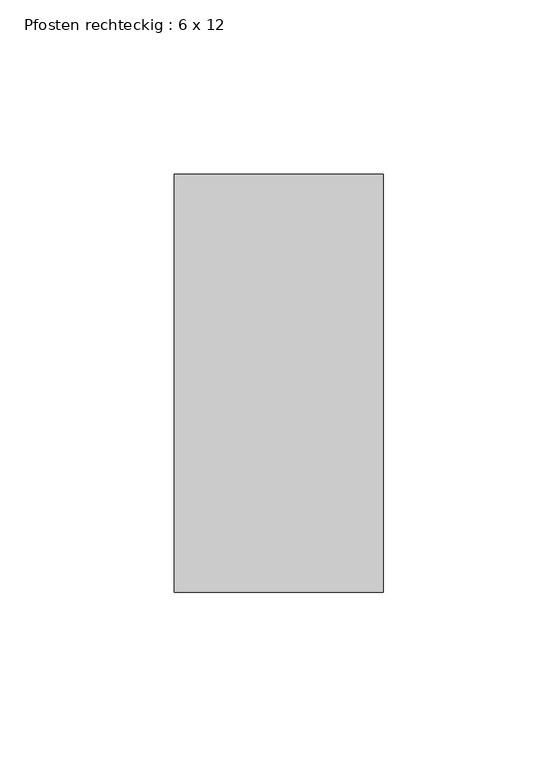
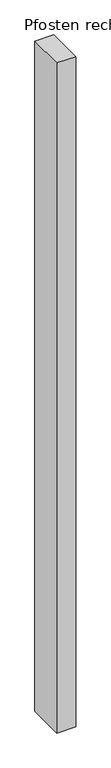
"""IFC4 building model written with IfcOpenShell, lengths in millimetres: member geometry, Pfosten rechteckig : 6 x 12."""

import ifcopenshell
import ifcopenshell.guid

model = None  # the IFC model being written
_history = None  # IfcOwnerHistory: only IFC2X3 demands one
_inside = {}  # id of a spatial element -> (the spatial element, [elements in it])
_under = {}  # id of a project, library or spatial element -> (it, [spatial elements below it])
_declared = {}  # id of a project -> (the project, [libraries it declares])
_typed = {}  # id of a type object -> (the type object, [elements of that type])
_made_of = {}  # id of a material, layer set ... -> (it, [elements and type objects made of it])


def new_model(schema):
    """Start an empty IFC model of exactly this schema.

    Asked for "IFC4X3", IfcOpenShell would pick the latest addendum, in which some entities
    have other attributes; the version numbers below select the first issue.
    IFC2X3 requires an IfcOwnerHistory on every rooted entity: one is made here for all.
    """
    global model, _history
    if schema == "IFC4X3":
        model = ifcopenshell.file(schema_version=(4, 3, 0, 0))
    else:
        model = ifcopenshell.file(schema=schema)
    _inside.clear()
    _under.clear()
    _declared.clear()
    _typed.clear()
    _made_of.clear()
    _history = None
    if model.schema == "IFC2X3":
        org = make("IfcOrganization", Name="unknown")
        user = make(
            "IfcPersonAndOrganization",
            ThePerson=make("IfcPerson", FamilyName="unknown"),
            TheOrganization=org,
        )
        app = make(
            "IfcApplication",
            ApplicationDeveloper=org,
            Version="unknown",
            ApplicationFullName="unknown",
            ApplicationIdentifier="unknown",
        )
        _history = make(
            "IfcOwnerHistory",
            OwningUser=user,
            OwningApplication=app,
            ChangeAction="ADDED",
            CreationDate=0,
        )
    return model


def make(cls, **values):
    """One entity of the class cls with the attributes given. An attribute that is None is left unset."""
    return model.create_entity(
        cls, **{name: value for name, value in values.items() if value is not None}
    )


def rooted(cls, **values):
    """An entity with a GlobalId (a new one), such as an element, a storey or a relation."""
    return make(cls, GlobalId=ifcopenshell.guid.new(), OwnerHistory=_history, **values)


def si_unit(unit_type, name, prefix=None):
    """IfcSIUnit, for example si_unit("LENGTHUNIT", "METRE", prefix="MILLI")."""
    return make("IfcSIUnit", UnitType=unit_type, Prefix=prefix, Name=name)


def assignment(units):
    """IfcUnitAssignment: the units of a project."""
    return None if units is None else make("IfcUnitAssignment", Units=units)


def point(xyz):
    """IfcCartesianPoint."""
    return None if xyz is None else make("IfcCartesianPoint", Coordinates=xyz)


def direction(xyz):
    """IfcDirection."""
    return None if xyz is None else make("IfcDirection", DirectionRatios=xyz)


def frame(location, z_axis=None, x_axis=None):
    """IfcAxis2Placement3D, a coordinate frame: its origin and axes. An axis left out is left unset."""
    return make(
        "IfcAxis2Placement3D",
        Location=point(location),
        Axis=direction(z_axis),
        RefDirection=direction(x_axis),
    )


def origin():
    """The frame at (0, 0, 0) with its axes left unset."""
    return frame((0.0, 0.0, 0.0))


def place(relative_to, where):
    """IfcLocalPlacement: puts the frame where relative to a parent placement (None: the world)."""
    return make(
        "IfcLocalPlacement", PlacementRelTo=relative_to, RelativePlacement=where
    )


def context(
    kind, dimensions, precision=None, world=None, true_north=None, identifier=None
):
    """IfcGeometricRepresentationContext, for example the 3D "Model" context."""
    return make(
        "IfcGeometricRepresentationContext",
        ContextIdentifier=identifier,
        ContextType=kind,
        CoordinateSpaceDimension=dimensions,
        Precision=precision,
        WorldCoordinateSystem=world,
        TrueNorth=true_north,
    )


def project(units=None, contexts=None):
    """IfcProject with its units and contexts."""
    return rooted(
        "IfcProject",
        Name="project",
        RepresentationContexts=contexts,
        UnitsInContext=assignment(units),
    )


def spatial(cls, under=None, at=None, **own):
    """A site, building, storey or space (cls), placed at a placement, below another one or the project."""
    s = rooted(cls, ObjectPlacement=at, **own)
    if under is not None:
        _under.setdefault(under.id(), (under, []))[1].append(s)
    return s


def polyline(points):
    """IfcPolyline through the points."""
    return make("IfcPolyline", Points=[point(p) for p in points])


def outline(outer, holes=None, kind="AREA"):
    """IfcArbitraryClosedProfileDef: a profile drawn as a closed curve; with holes, ...WithVoids."""
    if holes is None:
        return make("IfcArbitraryClosedProfileDef", ProfileType=kind, OuterCurve=outer)
    return make(
        "IfcArbitraryProfileDefWithVoids",
        ProfileType=kind,
        OuterCurve=outer,
        InnerCurves=holes,
    )


def extrude(swept, where, along, depth):
    """IfcExtrudedAreaSolid: the profile swept, set in the frame where, extruded along a direction by depth."""
    return make(
        "IfcExtrudedAreaSolid",
        SweptArea=swept,
        Position=where,
        ExtrudedDirection=direction(along),
        Depth=depth,
    )


def shape(context_of_items, identifier, shape_type, items):
    """IfcShapeRepresentation: the items that make up one representation, for example the "Body"."""
    return make(
        "IfcShapeRepresentation",
        ContextOfItems=context_of_items,
        RepresentationIdentifier=identifier,
        RepresentationType=shape_type,
        Items=items,
    )


def source(mapping_origin, context_of_items, identifier, shape_type, items):
    """IfcRepresentationMap: a shape defined once, which mapped items show again and again."""
    return make(
        "IfcRepresentationMap",
        MappingOrigin=mapping_origin,
        MappedRepresentation=shape(context_of_items, identifier, shape_type, items),
    )


def transform(
    local_origin,
    x_axis=None,
    y_axis=None,
    z_axis=None,
    scale=None,
    scale2=None,
    scale3=None,
    uniform=True,
):
    """IfcCartesianTransformationOperator3D, or its non-uniform kind. x_axis, y_axis, z_axis: its Axis1, 2, 3."""
    if uniform:
        return make(
            "IfcCartesianTransformationOperator3D",
            Axis1=direction(x_axis),
            Axis2=direction(y_axis),
            LocalOrigin=point(local_origin),
            Scale=scale,
            Axis3=direction(z_axis),
        )
    return make(
        "IfcCartesianTransformationOperator3DnonUniform",
        Axis1=direction(x_axis),
        Axis2=direction(y_axis),
        LocalOrigin=point(local_origin),
        Scale=scale,
        Axis3=direction(z_axis),
        Scale2=scale2,
        Scale3=scale3,
    )


def mapped(mapping_source, mapping_target):
    """IfcMappedItem: shows the shape of a source again, moved by a transform."""
    return make(
        "IfcMappedItem", MappingSource=mapping_source, MappingTarget=mapping_target
    )


def made_of(thing, what):
    """Note that an element or type object is made of a material, layer set ...; save() writes the relation."""
    if what is not None:
        _made_of.setdefault(what.id(), (what, []))[1].append(thing)
    return thing


def element(
    cls,
    number,
    at=None,
    inside=None,
    cuts=None,
    type_object=None,
    material=None,
    context=None,
    identifier="Body",
    shape_type=None,
    held_by="IfcProductDefinitionShape",
    body=None,
    shapes=None,
    **own,
):
    """One element of the class cls, such as IfcWall. Its Tag is "e" and its number.

    at: its placement. inside: the storey or other place that contains it. cuts: it is an
    opening in that element (IfcRelVoidsElement). A single representation is given by context,
    identifier, shape_type and body (its items); several are given by shapes. held_by: the class
    of the entity that holds the representations. save() writes the other relations.
    """
    e = rooted(cls, Tag="e%d" % number, ObjectPlacement=at, **own)
    if body is not None:
        shapes = [shape(context, identifier, shape_type, body)]
    if shapes is not None:
        e.Representation = make(held_by, Representations=shapes)
    if inside is not None:
        _inside.setdefault(inside.id(), (inside, []))[1].append(e)
    if cuts is not None:
        rooted(
            "IfcRelVoidsElement", RelatingBuildingElement=cuts, RelatedOpeningElement=e
        )
    if type_object is not None:
        _typed.setdefault(type_object.id(), (type_object, []))[1].append(e)
    return made_of(e, material)


def aggregate(whole, parts):
    """IfcRelAggregates: a whole, such as a stair, and the parts it consists of."""
    return rooted("IfcRelAggregates", RelatingObject=whole, RelatedObjects=parts)


def save(model, path):
    """Write the relations noted so far, then the file.

    IfcRelAggregates (storeys below a building ...), IfcRelContainedInSpatialStructure (elements
    in a storey), IfcRelDefinesByType, IfcRelAssociatesMaterial and IfcRelDeclares: one each for
    every whole, place, type object, material and project.
    """
    for whole, parts in _under.values():
        aggregate(whole, parts)
    for where, things in _inside.values():
        rooted(
            "IfcRelContainedInSpatialStructure",
            RelatedElements=things,
            RelatingStructure=where,
        )
    for kind, things in _typed.values():
        rooted("IfcRelDefinesByType", RelatedObjects=things, RelatingType=kind)
    for what, things in _made_of.values():
        rooted("IfcRelAssociatesMaterial", RelatedObjects=things, RelatingMaterial=what)
    for by, libraries in _declared.values():
        rooted("IfcRelDeclares", RelatingContext=by, RelatedDefinitions=libraries)
    model.write(path)


def pfosten_rechteckig_6_x_12_8f909f43(model_context):
    return source(origin(), model_context, "Body", "SweptSolid", [
        extrude(outline(polyline([(30.0, 60.0), (30.0, -60.0), (-30.0, -60.0), (-30.0, 60.0), (30.0, 60.0)])), frame((0.0, 0.0, -2250.0), z_axis=(0.0, 0.0, 1.0), x_axis=(1.0, 0.0, 0.0)), (0.0, 0.0, 1.0), 2250.0),
    ])


if __name__ == "__main__":
    model = new_model("IFC4")
    model_context = context("Model", 3, world=origin())
    ifc_project = project(units=[si_unit("LENGTHUNIT", "METRE", prefix="MILLI")], contexts=[model_context])
    site = spatial("IfcSite", under=ifc_project)
    building = spatial("IfcBuilding", under=site)
    placement = place(None, origin())
    pfosten_rechteckig_6_x_12_shape = pfosten_rechteckig_6_x_12_8f909f43(model_context)
    element("IfcMember", 1, ObjectType="Pfosten rechteckig : 6 x 12", at=placement, inside=building, context=model_context, shape_type="MappedRepresentation", body=[
        mapped(pfosten_rechteckig_6_x_12_shape, transform((0.0, 0.0, 0.0), x_axis=(1.0, 0.0, 0.0), y_axis=(0.0, 1.0, 0.0), z_axis=(0.0, 0.0, 1.0))),
    ])
    save(model, "model.ifc")

# Revit data of these elements
# Type "Pfosten rechteckig : 6 x 12"
#   built-in parameter 1007304 = 0.393701 (stored number, unit not read)
#   built-in parameter 1007301 = 0.0984252 (stored number, unit not read)
#   built-in parameter 1007300 = 0.0984252 (stored number, unit not read)
# Element 1 (IfcMember, "Pfosten rechteckig : 6 x 12")
#   Materials on its faces: "Metall - verzinkt"
# Materials
#   "Metall - verzinkt": class "Allgemeines", colour RGB 200 200 200, transparency 0, Cost = 0
